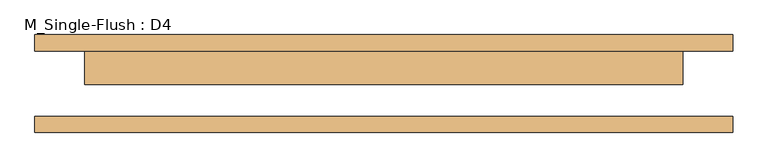
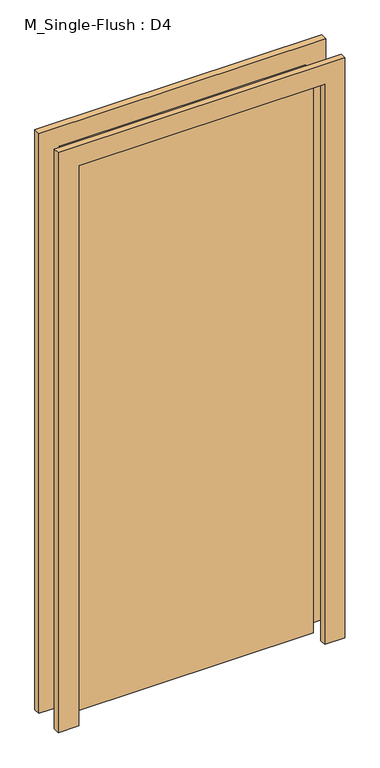
"""IFC4 building model written with IfcOpenShell, lengths in millimetres: door geometry, M_Single-Flush : D4."""

from ifc_helpers import new_model, si_unit, frame, origin, origin_with_axes, place, context, project, spatial, polyline, outline, extrude, source, transform, mapped, element, save


def m_single_flush_d4_9a91d6d9(model_context):
    return source(origin(), model_context, "Body", "SweptSolid", [
        extrude(outline(polyline([(2286.0, -534.5), (0.0, -534.5), (0.0, -458.5), (2210.0, -458.5), (2210.0, 458.5), (0.0, 458.5), (0.0, 534.5), (2286.0, 534.5), (2286.0, -534.5)])), frame((0.0, 50.0, 0.0), z_axis=(0.0, 1.0, 0.0), x_axis=(0.0, 0.0, 1.0)), (0.0, 0.0, 1.0), 25.0),
        extrude(outline(polyline([(2286.0, 534.5), (2286.0, -534.5), (0.0, -534.5), (0.0, -458.5), (2210.0, -458.5), (2210.0, 458.5), (0.0, 458.5), (0.0, 534.5), (2286.0, 534.5)])), frame((0.0, -75.0, 0.0), z_axis=(0.0, 1.0, 0.0), x_axis=(0.0, 0.0, 1.0)), (0.0, 0.0, 1.0), 25.0),
        extrude(outline(polyline([(458.5, -1.0), (-458.5, -1.0), (-458.5, 50.0), (458.5, 50.0), (458.5, -1.0)])), origin_with_axes(), (0.0, 0.0, 1.0), 2210.0),
    ])


if __name__ == "__main__":
    model = new_model("IFC4")
    model_context = context("Model", 3, world=origin())
    ifc_project = project(units=[si_unit("LENGTHUNIT", "METRE", prefix="MILLI")], contexts=[model_context])
    site = spatial("IfcSite", under=ifc_project)
    building = spatial("IfcBuilding", under=site)
    placement = place(None, origin())
    m_single_flush_d4_shape = m_single_flush_d4_9a91d6d9(model_context)
    element("IfcDoor", 1, ObjectType="M_Single-Flush : D4", at=placement, inside=building, context=model_context, shape_type="MappedRepresentation", body=[
        mapped(m_single_flush_d4_shape, transform((0.0, 0.0, 0.0), x_axis=(1.0, 0.0, 0.0), y_axis=(0.0, 1.0, 0.0), z_axis=(0.0, 0.0, 1.0))),
    ])
    save(model, "model.ifc")

# Revit data of these elements
# Type "M_Single-Flush : D4"
#   Type Mark = "21"
#   Thickness = 51 mm
#   Height = 2210 mm
#   Trim Projection Ext = 25 mm
#   Trim Projection Int = 25 mm
#   Trim Width = 76 mm
#   Width = 917 mm
#   Door Material = Door - Panel
#   Frame Material = Door - Frame
#   Function = (empty or 0)
#   Wall Closure = (empty or 0)
# Element 1 (IfcDoor, "M_Single-Flush : D4")
#   Materials on its faces: "Door - Frame", "Door - Panel"
# Materials
#   "Door - Panel": class "Wood", colour RGB 210 159 95, transparency 0
#   "Door - Frame": class "Miscellaneous", colour RGB 118 70 51, transparency 0
